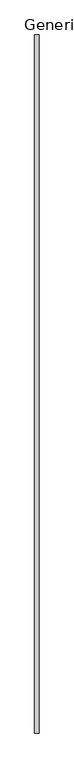
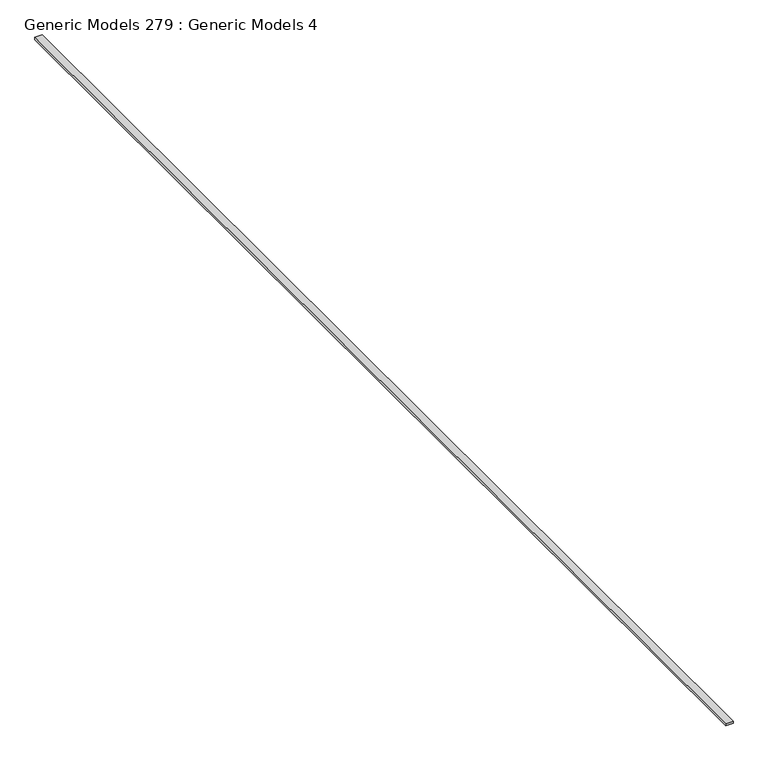
"""IFC4 building model written with IfcOpenShell, lengths in millimetres: proxy geometry, Generic Models 279 : Generic Models 4."""

from ifc_helpers import new_model, si_unit, frame, origin, place, context, project, spatial, polyline, outline, extrude, source, transform, mapped, element, save


def generic_models_279_generic_models_4_e5157994(model_context):
    return source(origin(), model_context, "Body", "SweptSolid", [
        extrude(outline(polyline([(35688.6626306, 12775.6158826), (35776.3520399, 12775.6158826), (35776.3520399, -1143.5841174), (35688.6626306, -1143.5841174), (35688.6626306, 12775.6158826)])), frame((0.0, 0.0, 129263.3128468), z_axis=(0.0, 0.0, 1.0), x_axis=(1.0, 0.0, 0.0)), (0.0, 0.0, 1.0), 27.8449747),
    ])


if __name__ == "__main__":
    model = new_model("IFC4")
    model_context = context("Model", 3, world=origin())
    ifc_project = project(units=[si_unit("LENGTHUNIT", "METRE", prefix="MILLI")], contexts=[model_context])
    site = spatial("IfcSite", under=ifc_project)
    building = spatial("IfcBuilding", under=site)
    placement = place(None, origin())
    generic_models_279_generic_models_4_shape = generic_models_279_generic_models_4_e5157994(model_context)
    element("IfcBuildingElementProxy", 1, Name="Generic Models 279 : Generic Models 4", ObjectType="Generic Models 279 : Generic Models 4", at=placement, inside=building, context=model_context, shape_type="MappedRepresentation", body=[
        mapped(generic_models_279_generic_models_4_shape, transform((0.0, 0.0, 0.0), x_axis=(1.0, 0.0, 0.0), y_axis=(0.0, 1.0, 0.0), z_axis=(0.0, 0.0, 1.0))),
    ])
    save(model, "model.ifc")

# Revit data of these elements
# Element 1 (IfcBuildingElementProxy, "Generic Models 279 : Generic Models 4")
#   Materials on its faces: "_BLOCKING AS REQUIRED"
# Materials
#   "_BLOCKING AS REQUIRED": class "Generic", colour RGB 177 130 114, transparency 0, Cost = 0
